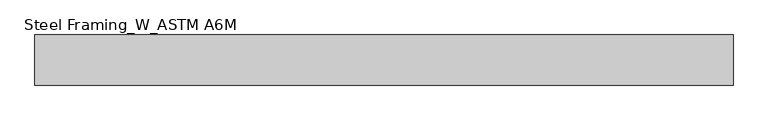
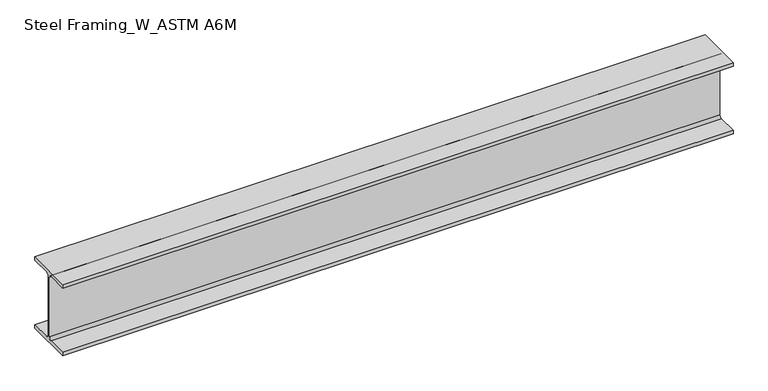
"""IFC4 building model written with IfcOpenShell, lengths in millimetres: beam geometry, Steel Framing_W_ASTM A6M : H_SB_AR_S02_W200x31.3_B6."""

from ifc_helpers import new_model, si_unit, point, frame, frame_2d, origin, place, context, project, spatial, polyline, circle_curve, trimmed, segment, composite_curve, outline, extrude, source, transform, mapped, element, save


def steel_framing_w_astm_a6m_892892c9(model_context):
    return source(origin(), model_context, "Body", "SweptSolid", [
        extrude(outline(composite_curve([segment(polyline([(67.0, -94.8), (67.0, -105.0), (-67.0, -105.0), (-67.0, -94.8), (-10.775, -94.8)]), True, "CONTINUOUS"), segment(trimmed(circle_curve(frame_2d((-10.775, -87.2)), 7.6), [point((-10.775, -94.8))], [point((-3.175, -87.2))], True, "CARTESIAN"), True, "CONTINUOUS"), segment(polyline([(-3.175, -87.2), (-3.175, 87.2)]), True, "CONTINUOUS"), segment(trimmed(circle_curve(frame_2d((-10.775, 87.2)), 7.6), [point((-3.175, 87.2))], [point((-10.775, 94.8))], True, "CARTESIAN"), True, "CONTINUOUS"), segment(polyline([(-10.775, 94.8), (-67.0, 94.8), (-67.0, 105.0), (67.0, 105.0), (67.0, 94.8), (10.775, 94.8)]), True, "CONTINUOUS"), segment(trimmed(circle_curve(frame_2d((10.775, 87.2)), 7.6), [point((10.775, 94.8))], [point((3.175, 87.2))], True, "CARTESIAN"), True, "CONTINUOUS"), segment(polyline([(3.175, 87.2), (3.175, -87.2)]), True, "CONTINUOUS"), segment(trimmed(circle_curve(frame_2d((10.775, -87.2)), 7.6), [point((3.175, -87.2))], [point((10.775, -94.8))], True, "CARTESIAN"), True, "CONTINUOUS"), segment(polyline([(10.775, -94.8), (67.0, -94.8)]), True, "CONTINUOUS")], self_intersect=False)), frame((-956.9, 0.0, 0.0), z_axis=(1.0, 0.0, 0.0), x_axis=(0.0, 1.0, 0.0)), (0.0, 0.0, 1.0), 1865.0),
    ])


if __name__ == "__main__":
    model = new_model("IFC4")
    model_context = context("Model", 3, world=origin())
    ifc_project = project(units=[si_unit("LENGTHUNIT", "METRE", prefix="MILLI")], contexts=[model_context])
    site = spatial("IfcSite", under=ifc_project)
    building = spatial("IfcBuilding", under=site)
    placement = place(None, origin())
    steel_framing_w_astm_a6m_shape = steel_framing_w_astm_a6m_892892c9(model_context)
    element("IfcBeam", 1, ObjectType="Steel Framing_W_ASTM A6M : H_SB_AR_S02_W200x31.3_B6", at=placement, inside=building, context=model_context, shape_type="MappedRepresentation", body=[
        mapped(steel_framing_w_astm_a6m_shape, transform((0.0, 0.0, 0.0), x_axis=(1.0, 0.0, 0.0), y_axis=(0.0, 1.0, 0.0), z_axis=(0.0, 0.0, 1.0))),
    ])
    save(model, "model.ifc")

# Revit data of these elements
# Type "Steel Framing_W_ASTM A6M : H_SB_AR_S02_W200x31.3_B6"
#   Type Mark = "B6"
#   Section Name Key = "W8x21"
#   Width = 13.4 cm
#   Web Thickness = 0.635 cm
#   Web Fillet = 0.76 cm
#   Warping Constant = 40800.0 cm⁶
#   Torsional Moment of Inertia = 11.70 cm⁴
#   Section Area = 39.7 cm²
#   Plastic Modulus weak axis = 93.2 cm³
#   Plastic Modulus strong axis = 334.0 cm³
#   Perimeter = 0.93 m²/m
#   Nominal Weight = 31.30 kgf/m
#   Moment of Inertia weak axis = 407.00 cm⁴
#   Moment of Inertia strong axis = 3130.00 cm⁴
#   Height = 21.0 cm
#   Flange Thickness = 1.02 cm
#   Elastic Modulus weak axis = 60.8 cm³
#   Elastic Modulus strong axis = 298.0 cm³
#   Centroid Vertical = 10.5 cm
#   Centroid Horizontal = 6.7 cm
#   Length [instance default] = 1500 mm
#   Structural Material [instance default] = Steel, 45-345
#   Bolt Spacing = 0
#   Assembly Code = ""
# Element 1 (IfcBeam, "Steel Framing_W_ASTM A6M : H_SB_AR_S02_W200x31.3_B6")
#   Materials on its faces: "Steel, 45-345"
# Materials
#   "Steel, 45-345": class "Metal", colour RGB 189 187 185, transparency 0, Description = "Steel 345 MPa", Cost = 0
